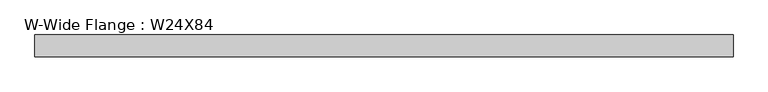
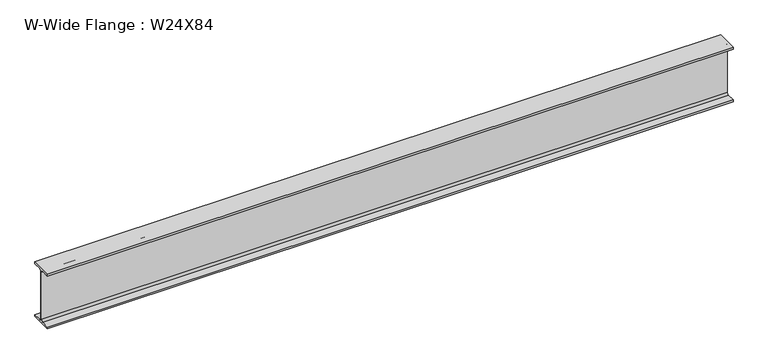
"""IFC4 building model written with IfcOpenShell, lengths in millimetres: beam geometry, W-Wide Flange : W24X84."""

from ifc_helpers import new_model, si_unit, point, frame, frame_2d, origin, place, context, project, spatial, polyline, circle_curve, trimmed, segment, composite_curve, outline, extrude, source, transform, mapped, element, save


def w_wide_flange_w24x84_0eef56af(model_context):
    return source(origin(), model_context, "Body", "SweptSolid", [
        extrude(outline(composite_curve([segment(polyline([(114.554, -286.512), (114.554, -306.07), (-114.554, -306.07), (-114.554, -286.512), (-29.2735, -286.512)]), True, "CONTINUOUS"), segment(trimmed(circle_curve(frame_2d((-29.2735, -263.2075)), 23.3045), [point((-29.2735, -286.512))], [point((-5.969, -263.2075))], True, "CARTESIAN"), True, "CONTINUOUS"), segment(polyline([(-5.969, -263.2075), (-5.969, 263.2075)]), True, "CONTINUOUS"), segment(trimmed(circle_curve(frame_2d((-29.2735, 263.2075)), 23.3045), [point((-5.969, 263.2075))], [point((-29.2735, 286.512))], True, "CARTESIAN"), True, "CONTINUOUS"), segment(polyline([(-29.2735, 286.512), (-114.554, 286.512), (-114.554, 306.07), (114.554, 306.07), (114.554, 286.512), (29.2735, 286.512)]), True, "CONTINUOUS"), segment(trimmed(circle_curve(frame_2d((29.2735, 263.2075)), 23.3045), [point((29.2735, 286.512))], [point((5.969, 263.2075))], True, "CARTESIAN"), True, "CONTINUOUS"), segment(polyline([(5.969, 263.2075), (5.969, -263.2075)]), True, "CONTINUOUS"), segment(trimmed(circle_curve(frame_2d((29.2735, -263.2075)), 23.3045), [point((5.969, -263.2075))], [point((29.2735, -286.512))], True, "CARTESIAN"), True, "CONTINUOUS"), segment(polyline([(29.2735, -286.512), (114.554, -286.512)]), True, "CONTINUOUS")], self_intersect=False)), frame((-3645.6441406, 0.0, 0.0), z_axis=(1.0, 0.0, 0.0), x_axis=(0.0, 1.0, 0.0)), (0.0, 0.0, 1.0), 7291.2882813),
    ])


if __name__ == "__main__":
    model = new_model("IFC4")
    model_context = context("Model", 3, world=origin())
    ifc_project = project(units=[si_unit("LENGTHUNIT", "METRE", prefix="MILLI")], contexts=[model_context])
    site = spatial("IfcSite", under=ifc_project)
    building = spatial("IfcBuilding", under=site)
    placement = place(None, origin())
    w_wide_flange_w24x84_shape = w_wide_flange_w24x84_0eef56af(model_context)
    element("IfcBeam", 1, ObjectType="W-Wide Flange : W24X84", at=placement, inside=building, context=model_context, shape_type="MappedRepresentation", body=[
        mapped(w_wide_flange_w24x84_shape, transform((0.0, 0.0, 0.0), x_axis=(1.0, 0.0, 0.0), y_axis=(0.0, 1.0, 0.0), z_axis=(0.0, 0.0, 1.0))),
    ])
    save(model, "model.ifc")

# Revit data of these elements
# Type "W-Wide Flange : W24X84"
#   Assembly Code = "B10"
#   W = 84
#   Length [instance default] = 1524 mm
#   bf = 229.108 mm
#   d = 612.14 mm
#   k = 42.863 mm
#   k2 = 23.305 mm
#   tf = 19.558 mm
#   tw = 11.938 mm
#   A = 0.0159355 m²
#   Structural Material [instance default] = Steel ASTM A992
# Element 1 (IfcBeam, "W-Wide Flange : W24X84")
#   Structural Material = Aluminum, Anodized Red
#   Materials on its faces: "Aluminum, Anodized Red"
# Materials
#   "Steel ASTM A992": class "Metal", colour RGB 128 0 0, transparency 0, Description = "Structural steel 50ksi", Cost = 0
#   "Aluminum, Anodized Red": class "Metal", colour RGB 120 120 120, transparency 0, Description = "Anodized aluminum, red", Cost = 0
